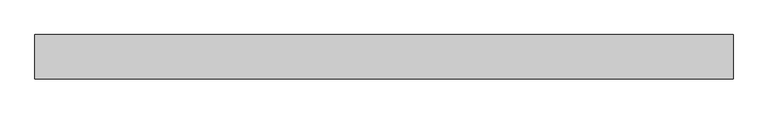
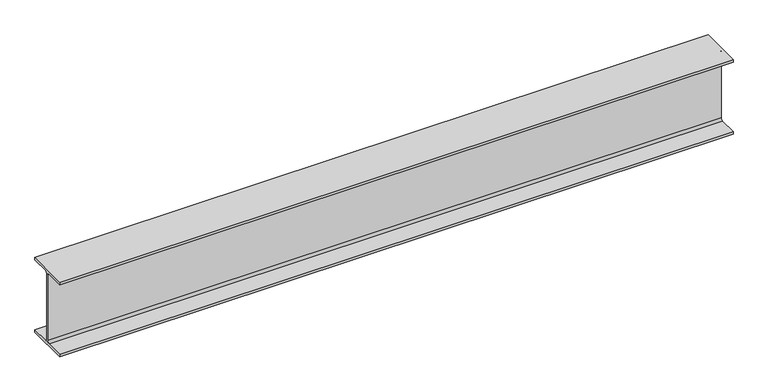
"""IFC4 building model written with IfcOpenShell, lengths in millimetres: beam geometry, Steel Beam_H-KSD3502 : H_SB_ASB_H-250x125x6x9."""

from ifc_helpers import new_model, si_unit, point, frame, frame_2d, origin, place, context, project, spatial, polyline, circle_curve, trimmed, segment, composite_curve, outline, extrude, source, transform, mapped, element, save


def beam_59f19b17(model_context):
    return source(origin(), model_context, "Body", "SweptSolid", [
        extrude(outline(composite_curve([segment(polyline([(82.5, -141.5), (82.5, -151.7), (-82.5, -151.7), (-82.5, -141.5), (-11.9, -141.5)]), True, "CONTINUOUS"), segment(trimmed(circle_curve(frame_2d((-11.9, -132.6)), 8.9), [point((-11.9, -141.5))], [point((-3.0, -132.6))], True, "CARTESIAN"), True, "CONTINUOUS"), segment(polyline([(-3.0, -132.6), (-3.0, 132.6)]), True, "CONTINUOUS"), segment(trimmed(circle_curve(frame_2d((-11.9, 132.6)), 8.9), [point((-3.0, 132.6))], [point((-11.9, 141.5))], True, "CARTESIAN"), True, "CONTINUOUS"), segment(polyline([(-11.9, 141.5), (-82.5, 141.5), (-82.5, 151.7), (82.5, 151.7), (82.5, 141.5), (11.9, 141.5)]), True, "CONTINUOUS"), segment(trimmed(circle_curve(frame_2d((11.9, 132.6)), 8.9), [point((11.9, 141.5))], [point((3.0, 132.6))], True, "CARTESIAN"), True, "CONTINUOUS"), segment(polyline([(3.0, 132.6), (3.0, -132.6)]), True, "CONTINUOUS"), segment(trimmed(circle_curve(frame_2d((11.9, -132.6)), 8.9), [point((3.0, -132.6))], [point((11.9, -141.5))], True, "CARTESIAN"), True, "CONTINUOUS"), segment(polyline([(11.9, -141.5), (82.5, -141.5)]), True, "CONTINUOUS")], self_intersect=False)), frame((-1249.3, 0.0, 0.0), z_axis=(1.0, 0.0, 0.0), x_axis=(0.0, 1.0, 0.0)), (0.0, 0.0, 1.0), 2586.6),
    ])


if __name__ == "__main__":
    model = new_model("IFC4")
    model_context = context("Model", 3, world=origin())
    ifc_project = project(units=[si_unit("LENGTHUNIT", "METRE", prefix="MILLI")], contexts=[model_context])
    site = spatial("IfcSite", under=ifc_project)
    building = spatial("IfcBuilding", under=site)
    placement = place(None, origin())
    beam_shape = beam_59f19b17(model_context)
    element("IfcBeam", 1, ObjectType="Steel Beam_H-KSD3502 : H_SB_ASB_H-250x125x6x9", at=placement, inside=building, context=model_context, shape_type="MappedRepresentation", body=[
        mapped(beam_shape, transform((0.0, 0.0, 0.0), x_axis=(1.0, 0.0, 0.0), y_axis=(0.0, 1.0, 0.0), z_axis=(0.0, 0.0, 1.0))),
    ])
    save(model, "model.ifc")

# Revit data of these elements
# Type "Steel Beam_H-KSD3502 : H_SB_ASB_H-250x125x6x9"
#   Width = 12.5 cm
#   Web Thickness = 0.6 cm
#   Web Fillet = 1.2 cm
#   Warping Constant = 42539.8 cm⁶
#   Torsional Moment of Inertia = 7.8102 cm⁴
#   Torsional Modulus = 1.0 cm³
#   Section Area = 37.66 cm²
#   Plastic Modulus weak axis = 73.1 cm³
#   Plastic Modulus strong axis = 366.0 cm³
#   Perimeter = 0.97 m²/m
#   Nominal Weight = 29.60 kgf/m
#   Moment of Inertia weak axis = 294.00 cm⁴
#   Moment of Inertia strong axis = 4050.00 cm⁴
#   Height = 25.0 cm
#   Flange Thickness = 0.9 cm
#   Elastic Modulus weak axis = 47.0 cm³
#   Elastic Modulus strong axis = 324.0 cm³
#   Centroid Vertical = 12.5 cm
#   Centroid Horizontal = 6.25 cm
#   Length [instance default] = 1.5240 m
#   Structural Material [instance default] = Steel, 45-345
#   Assembly Code = ""
# Element 1 (IfcBeam, "Steel Beam_H-KSD3502 : H_SB_ASB_H-250x125x6x9")
#   Structural Material = none
# Materials
#   "Steel, 45-345": class "Metal", colour RGB 189 187 185, transparency 0, Description = "Steel 345 MPa", Cost = 0
